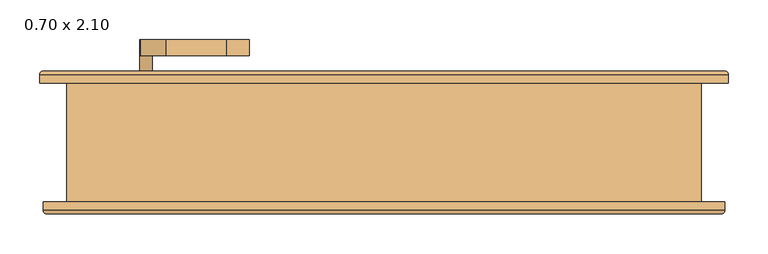
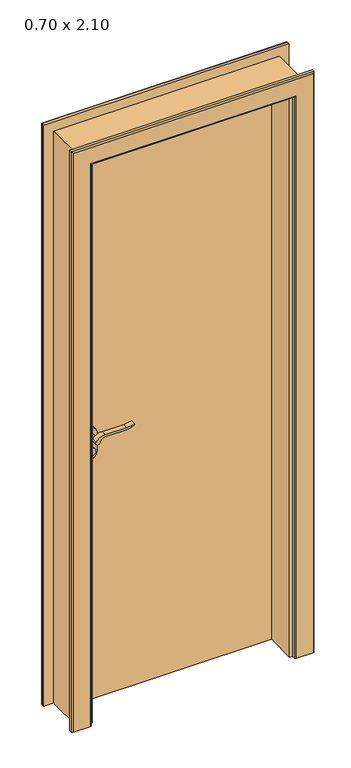
"""IFC4 building model written with IfcOpenShell, lengths in millimetres: door geometry, PORTA_DE_ABRIR_MADEIRA : 0.70 x 2.10."""

import ifcopenshell
import ifcopenshell.guid

model = None  # the IFC model being written
_history = None  # IfcOwnerHistory: only IFC2X3 demands one
_inside = {}  # id of a spatial element -> (the spatial element, [elements in it])
_under = {}  # id of a project, library or spatial element -> (it, [spatial elements below it])
_declared = {}  # id of a project -> (the project, [libraries it declares])
_typed = {}  # id of a type object -> (the type object, [elements of that type])
_made_of = {}  # id of a material, layer set ... -> (it, [elements and type objects made of it])


def new_model(schema):
    """Start an empty IFC model of exactly this schema.

    Asked for "IFC4X3", IfcOpenShell would pick the latest addendum, in which some entities
    have other attributes; the version numbers below select the first issue.
    IFC2X3 requires an IfcOwnerHistory on every rooted entity: one is made here for all.
    """
    global model, _history
    if schema == "IFC4X3":
        model = ifcopenshell.file(schema_version=(4, 3, 0, 0))
    else:
        model = ifcopenshell.file(schema=schema)
    _inside.clear()
    _under.clear()
    _declared.clear()
    _typed.clear()
    _made_of.clear()
    _history = None
    if model.schema == "IFC2X3":
        org = make("IfcOrganization", Name="unknown")
        user = make(
            "IfcPersonAndOrganization",
            ThePerson=make("IfcPerson", FamilyName="unknown"),
            TheOrganization=org,
        )
        app = make(
            "IfcApplication",
            ApplicationDeveloper=org,
            Version="unknown",
            ApplicationFullName="unknown",
            ApplicationIdentifier="unknown",
        )
        _history = make(
            "IfcOwnerHistory",
            OwningUser=user,
            OwningApplication=app,
            ChangeAction="ADDED",
            CreationDate=0,
        )
    return model


def make(cls, **values):
    """One entity of the class cls with the attributes given. An attribute that is None is left unset."""
    return model.create_entity(
        cls, **{name: value for name, value in values.items() if value is not None}
    )


def rooted(cls, **values):
    """An entity with a GlobalId (a new one), such as an element, a storey or a relation."""
    return make(cls, GlobalId=ifcopenshell.guid.new(), OwnerHistory=_history, **values)


def si_unit(unit_type, name, prefix=None):
    """IfcSIUnit, for example si_unit("LENGTHUNIT", "METRE", prefix="MILLI")."""
    return make("IfcSIUnit", UnitType=unit_type, Prefix=prefix, Name=name)


def assignment(units):
    """IfcUnitAssignment: the units of a project."""
    return None if units is None else make("IfcUnitAssignment", Units=units)


def point(xyz):
    """IfcCartesianPoint."""
    return None if xyz is None else make("IfcCartesianPoint", Coordinates=xyz)


def direction(xyz):
    """IfcDirection."""
    return None if xyz is None else make("IfcDirection", DirectionRatios=xyz)


def frame(location, z_axis=None, x_axis=None):
    """IfcAxis2Placement3D, a coordinate frame: its origin and axes. An axis left out is left unset."""
    return make(
        "IfcAxis2Placement3D",
        Location=point(location),
        Axis=direction(z_axis),
        RefDirection=direction(x_axis),
    )


def frame_2d(location, x_axis=None):
    """IfcAxis2Placement2D, a coordinate frame in the plane: its origin and x axis."""
    return make(
        "IfcAxis2Placement2D", Location=point(location), RefDirection=direction(x_axis)
    )


def origin():
    """The frame at (0, 0, 0) with its axes left unset."""
    return frame((0.0, 0.0, 0.0))


def origin_with_axes():
    """The frame at (0, 0, 0) with the z axis (0, 0, 1) and the x axis (1, 0, 0) written out."""
    return frame((0.0, 0.0, 0.0), z_axis=(0.0, 0.0, 1.0), x_axis=(1.0, 0.0, 0.0))


def place(relative_to, where):
    """IfcLocalPlacement: puts the frame where relative to a parent placement (None: the world)."""
    return make(
        "IfcLocalPlacement", PlacementRelTo=relative_to, RelativePlacement=where
    )


def context(
    kind, dimensions, precision=None, world=None, true_north=None, identifier=None
):
    """IfcGeometricRepresentationContext, for example the 3D "Model" context."""
    return make(
        "IfcGeometricRepresentationContext",
        ContextIdentifier=identifier,
        ContextType=kind,
        CoordinateSpaceDimension=dimensions,
        Precision=precision,
        WorldCoordinateSystem=world,
        TrueNorth=true_north,
    )


def project(units=None, contexts=None):
    """IfcProject with its units and contexts."""
    return rooted(
        "IfcProject",
        Name="project",
        RepresentationContexts=contexts,
        UnitsInContext=assignment(units),
    )


def spatial(cls, under=None, at=None, **own):
    """A site, building, storey or space (cls), placed at a placement, below another one or the project."""
    s = rooted(cls, ObjectPlacement=at, **own)
    if under is not None:
        _under.setdefault(under.id(), (under, []))[1].append(s)
    return s


def polyline(points):
    """IfcPolyline through the points."""
    return make("IfcPolyline", Points=[point(p) for p in points])


def circle_curve(where, radius):
    """IfcCircle in the frame where."""
    return make("IfcCircle", Position=where, Radius=radius)


def ellipse_curve(where, semi_axis1, semi_axis2):
    """IfcEllipse in the frame where."""
    return make(
        "IfcEllipse", Position=where, SemiAxis1=semi_axis1, SemiAxis2=semi_axis2
    )


def trimmed(basis, trim1, trim2, sense, master):
    """IfcTrimmedCurve: the piece of a basis curve between two trims."""
    return make(
        "IfcTrimmedCurve",
        BasisCurve=basis,
        Trim1=trim1,
        Trim2=trim2,
        SenseAgreement=sense,
        MasterRepresentation=master,
    )


def segment(curve, same_sense, transition):
    """IfcCompositeCurveSegment."""
    return make(
        "IfcCompositeCurveSegment",
        Transition=transition,
        SameSense=same_sense,
        ParentCurve=curve,
    )


def composite_curve(segments, self_intersect=None):
    """IfcCompositeCurve: segments joined end to end."""
    return make("IfcCompositeCurve", Segments=segments, SelfIntersect=self_intersect)


def outline(outer, holes=None, kind="AREA"):
    """IfcArbitraryClosedProfileDef: a profile drawn as a closed curve; with holes, ...WithVoids."""
    if holes is None:
        return make("IfcArbitraryClosedProfileDef", ProfileType=kind, OuterCurve=outer)
    return make(
        "IfcArbitraryProfileDefWithVoids",
        ProfileType=kind,
        OuterCurve=outer,
        InnerCurves=holes,
    )


def extrude(swept, where, along, depth):
    """IfcExtrudedAreaSolid: the profile swept, set in the frame where, extruded along a direction by depth."""
    return make(
        "IfcExtrudedAreaSolid",
        SweptArea=swept,
        Position=where,
        ExtrudedDirection=direction(along),
        Depth=depth,
    )


def faces_of(points, faces, orient=None, outer=None):
    """IfcFace entities. A face is a list of loops; a loop is a list of indices into points, from 0.

    orient and outer hold one flag for each loop. By default every Orientation is true, the
    first loop of a face is its IfcFaceOuterBound and the others are IfcFaceBound.
    """
    made = []
    for i, loops in enumerate(faces):
        bounds = []
        for j, loop in enumerate(loops):
            is_outer = j == 0 if outer is None else outer[i][j]
            bounds.append(
                make(
                    "IfcFaceOuterBound" if is_outer else "IfcFaceBound",
                    Bound=make("IfcPolyLoop", Polygon=[points[k] for k in loop]),
                    Orientation=True if orient is None else orient[i][j],
                )
            )
        made.append(make("IfcFace", Bounds=bounds))
    return made


def faceted_brep(points, faces, orient=None, outer=None, voids=None):
    """IfcFacetedBrep: a solid bounded by flat faces; with voids (closed shells), ...WithVoids."""
    shared = [point(p) for p in points]
    hull = make("IfcClosedShell", CfsFaces=faces_of(shared, faces, orient, outer))
    if voids is None:
        return make("IfcFacetedBrep", Outer=hull)
    return make(
        "IfcFacetedBrepWithVoids",
        Outer=hull,
        Voids=[
            make(cls, CfsFaces=faces_of(shared, fs, o, b)) for cls, fs, o, b in voids
        ],
    )


def shape(context_of_items, identifier, shape_type, items):
    """IfcShapeRepresentation: the items that make up one representation, for example the "Body"."""
    return make(
        "IfcShapeRepresentation",
        ContextOfItems=context_of_items,
        RepresentationIdentifier=identifier,
        RepresentationType=shape_type,
        Items=items,
    )


def source(mapping_origin, context_of_items, identifier, shape_type, items):
    """IfcRepresentationMap: a shape defined once, which mapped items show again and again."""
    return make(
        "IfcRepresentationMap",
        MappingOrigin=mapping_origin,
        MappedRepresentation=shape(context_of_items, identifier, shape_type, items),
    )


def transform(
    local_origin,
    x_axis=None,
    y_axis=None,
    z_axis=None,
    scale=None,
    scale2=None,
    scale3=None,
    uniform=True,
):
    """IfcCartesianTransformationOperator3D, or its non-uniform kind. x_axis, y_axis, z_axis: its Axis1, 2, 3."""
    if uniform:
        return make(
            "IfcCartesianTransformationOperator3D",
            Axis1=direction(x_axis),
            Axis2=direction(y_axis),
            LocalOrigin=point(local_origin),
            Scale=scale,
            Axis3=direction(z_axis),
        )
    return make(
        "IfcCartesianTransformationOperator3DnonUniform",
        Axis1=direction(x_axis),
        Axis2=direction(y_axis),
        LocalOrigin=point(local_origin),
        Scale=scale,
        Axis3=direction(z_axis),
        Scale2=scale2,
        Scale3=scale3,
    )


def mapped(mapping_source, mapping_target):
    """IfcMappedItem: shows the shape of a source again, moved by a transform."""
    return make(
        "IfcMappedItem", MappingSource=mapping_source, MappingTarget=mapping_target
    )


def made_of(thing, what):
    """Note that an element or type object is made of a material, layer set ...; save() writes the relation."""
    if what is not None:
        _made_of.setdefault(what.id(), (what, []))[1].append(thing)
    return thing


def element(
    cls,
    number,
    at=None,
    inside=None,
    cuts=None,
    type_object=None,
    material=None,
    context=None,
    identifier="Body",
    shape_type=None,
    held_by="IfcProductDefinitionShape",
    body=None,
    shapes=None,
    **own,
):
    """One element of the class cls, such as IfcWall. Its Tag is "e" and its number.

    at: its placement. inside: the storey or other place that contains it. cuts: it is an
    opening in that element (IfcRelVoidsElement). A single representation is given by context,
    identifier, shape_type and body (its items); several are given by shapes. held_by: the class
    of the entity that holds the representations. save() writes the other relations.
    """
    e = rooted(cls, Tag="e%d" % number, ObjectPlacement=at, **own)
    if body is not None:
        shapes = [shape(context, identifier, shape_type, body)]
    if shapes is not None:
        e.Representation = make(held_by, Representations=shapes)
    if inside is not None:
        _inside.setdefault(inside.id(), (inside, []))[1].append(e)
    if cuts is not None:
        rooted(
            "IfcRelVoidsElement", RelatingBuildingElement=cuts, RelatedOpeningElement=e
        )
    if type_object is not None:
        _typed.setdefault(type_object.id(), (type_object, []))[1].append(e)
    return made_of(e, material)


def aggregate(whole, parts):
    """IfcRelAggregates: a whole, such as a stair, and the parts it consists of."""
    return rooted("IfcRelAggregates", RelatingObject=whole, RelatedObjects=parts)


def save(model, path):
    """Write the relations noted so far, then the file.

    IfcRelAggregates (storeys below a building ...), IfcRelContainedInSpatialStructure (elements
    in a storey), IfcRelDefinesByType, IfcRelAssociatesMaterial and IfcRelDeclares: one each for
    every whole, place, type object, material and project.
    """
    for whole, parts in _under.values():
        aggregate(whole, parts)
    for where, things in _inside.values():
        rooted(
            "IfcRelContainedInSpatialStructure",
            RelatedElements=things,
            RelatingStructure=where,
        )
    for kind, things in _typed.values():
        rooted("IfcRelDefinesByType", RelatedObjects=things, RelatingType=kind)
    for what, things in _made_of.values():
        rooted("IfcRelAssociatesMaterial", RelatedObjects=things, RelatingMaterial=what)
    for by, libraries in _declared.values():
        rooted("IfcRelDeclares", RelatingContext=by, RelatedDefinitions=libraries)
    model.write(path)


def plane_surface(at):
    """IfcPlane: the flat surface through the origin of the frame at, square to its z axis."""
    return make("IfcPlane", Position=at)


def cylinder_surface(at, radius):
    """IfcCylindricalSurface: all points at the distance radius from the z axis of the frame at."""
    return make("IfcCylindricalSurface", Position=at, Radius=radius)


def advanced_brep(points, edges, surfaces, faces):
    """IfcAdvancedBrep: a solid bounded by faces that lie on surfaces and meet in shared edges.

    An edge is (start, end): straight between two places in points (the first is 0);
    or (start, end, curve); or (start, end, curve, False) where it runs against its curve.
    A face is (place in surfaces, loops), or (place, loops, False) where it looks against
    its surface's normal. A loop lists edges by number (the first is 1), with a minus sign
    where the edge is run from its end to its start. The first loop is the outer one.
    """
    corners = [point(p) for p in points]
    vertices = [make("IfcVertexPoint", VertexGeometry=c) for c in corners]
    made = []
    for start, end, *more in edges:
        made.append(
            make(
                "IfcEdgeCurve",
                EdgeStart=vertices[start],
                EdgeEnd=vertices[end],
                EdgeGeometry=more[0] if more else make("IfcPolyline", Points=[corners[start], corners[end]]),
                SameSense=more[1] if len(more) > 1 else True,
            )
        )
    hull = []
    for where, loops, *sense in faces:
        bounds = []
        for j, loop in enumerate(loops):
            ring = [make("IfcOrientedEdge", EdgeElement=made[abs(k) - 1], Orientation=k > 0) for k in loop]
            bounds.append(
                make(
                    "IfcFaceOuterBound" if j == 0 else "IfcFaceBound",
                    Bound=make("IfcEdgeLoop", EdgeList=ring),
                    Orientation=True,
                )
            )
        hull.append(make("IfcAdvancedFace", Bounds=bounds, FaceSurface=surfaces[where], SameSense=sense[0] if sense else True))
    return make("IfcAdvancedBrep", Outer=make("IfcClosedShell", CfsFaces=hull))


def door_0_70_x_2_10_357bc0c5(model_context):
    return source(origin(), model_context, "Body", "SolidModel", [
        extrude(outline(composite_curve([segment(trimmed(circle_curve(frame_2d((940.0, -300.0)), 15.0), [point((940.0, -285.0))], [point((940.0, -315.0))], False, "CARTESIAN"), True, "CONTINUOUS"), segment(trimmed(circle_curve(frame_2d((940.0, -300.0)), 15.0), [point((940.0, -315.0))], [point((940.0, -285.0))], False, "CARTESIAN"), True, "CONTINUOUS")], self_intersect=False)), frame((0.0, 15.0, 0.0), z_axis=(0.0, 1.0, 0.0), x_axis=(0.0, 0.0, 1.0)), (0.0, 0.0, 1.0), 10.0),
        extrude(outline(composite_curve([segment(trimmed(circle_curve(frame_2d((940.0, -300.0)), 15.0), [point((940.0, -285.0))], [point((940.0, -315.0))], False, "CARTESIAN"), True, "CONTINUOUS"), segment(trimmed(circle_curve(frame_2d((940.0, -300.0)), 15.0), [point((940.0, -315.0))], [point((940.0, -285.0))], False, "CARTESIAN"), True, "CONTINUOUS")], self_intersect=False)), frame((0.0, 80.0, 0.0), z_axis=(0.0, 1.0, 0.0), x_axis=(0.0, 0.0, 1.0)), (0.0, 0.0, 1.0), 10.0),
        extrude(outline(composite_curve([segment(trimmed(circle_curve(frame_2d((1000.0, -300.0)), 8.0), [point((1004.6523287, -306.5081363))], [point((1000.0, -292.0))], False, "CARTESIAN"), True, "CONTINUOUS"), segment(trimmed(circle_curve(frame_2d((994.8738613, -274.6138099)), 18.1261387), [point((1000.0, -292.0))], [point((1013.0, -274.6138099))], True, "CARTESIAN"), True, "CONTINUOUS"), segment(polyline([(1013.0, -274.6138099), (1013.0, -198.3564091)]), True, "CONTINUOUS"), segment(trimmed(circle_curve(frame_2d((1072.2709207, -201.9396612)), 59.3791355), [point((1013.0, -198.3564091))], [point((1022.2135558, -170.0))], False, "CARTESIAN"), True, "CONTINUOUS"), segment(polyline([(1022.2135558, -170.0), (1025.0, -170.0)]), True, "CONTINUOUS"), segment(trimmed(circle_curve(frame_2d((1103.2850638, -198.4227909)), 83.2850902), [point((1025.0, -170.0))], [point((1020.0, -198.3564091))], True, "CARTESIAN"), True, "CONTINUOUS"), segment(polyline([(1020.0, -198.3564091), (1020.0, -274.6325667)]), True, "CONTINUOUS"), segment(trimmed(circle_curve(frame_2d((982.7555521, -276.3324871)), 37.2832219), [point((1020.0, -274.6325667))], [point((1004.6523287, -306.5081363))], False, "CARTESIAN"), True, "CONTINUOUS")], self_intersect=False)), frame((0.0, -25.0, 0.0), z_axis=(0.0, 1.0, 0.0), x_axis=(0.0, 0.0, 1.0)), (0.0, 0.0, 1.0), 20.0),
        extrude(outline(composite_curve([segment(trimmed(circle_curve(frame_2d((994.8738682, -274.6138122)), 18.1261318), [point((999.9999903, -292.0))], [point((1013.0, -274.6138122))], True, "CARTESIAN"), True, "CONTINUOUS"), segment(polyline([(1013.0, -274.6138122), (1013.0, -198.3564091)]), True, "CONTINUOUS"), segment(trimmed(circle_curve(frame_2d((1072.2709207, -201.9396612)), 59.3791355), [point((1013.0, -198.3564091))], [point((1022.2135558, -170.0))], False, "CARTESIAN"), True, "CONTINUOUS"), segment(polyline([(1022.2135558, -170.0), (1025.0, -170.0)]), True, "CONTINUOUS"), segment(trimmed(circle_curve(frame_2d((1103.2850638, -198.4227909)), 83.2850902), [point((1025.0, -170.0))], [point((1020.0, -198.3564091))], True, "CARTESIAN"), True, "CONTINUOUS"), segment(polyline([(1020.0, -198.3564091), (1020.0, -274.6325667)]), True, "CONTINUOUS"), segment(trimmed(circle_curve(frame_2d((982.7555521, -276.3324871)), 37.2832219), [point((1020.0, -274.6325667))], [point((1004.6523287, -306.5081363))], False, "CARTESIAN"), True, "CONTINUOUS"), segment(trimmed(circle_curve(frame_2d((1000.0, -300.0)), 8.0), [point((1004.6523287, -306.5081363))], [point((999.9999903, -292.0))], False, "CARTESIAN"), True, "CONTINUOUS")], self_intersect=False)), frame((0.0, 110.0, 0.0), z_axis=(0.0, 1.0, 0.0), x_axis=(0.0, 0.0, 1.0)), (0.0, 0.0, 1.0), 20.0),
        extrude(outline(composite_curve([segment(trimmed(circle_curve(frame_2d((1000.0, -300.0)), 8.0), [point((1000.0, -292.0))], [point((1000.0, -308.0))], False, "CARTESIAN"), True, "CONTINUOUS"), segment(trimmed(circle_curve(frame_2d((1000.0, -300.0)), 8.0), [point((1000.0, -308.0))], [point((1000.0, -292.0))], False, "CARTESIAN"), True, "CONTINUOUS")], self_intersect=False)), frame((0.0, -5.0, 0.0), z_axis=(0.0, 1.0, 0.0), x_axis=(0.0, 0.0, 1.0)), (0.0, 0.0, 1.0), 30.0),
        extrude(outline(composite_curve([segment(trimmed(circle_curve(frame_2d((1000.0, -300.0)), 8.0), [point((1000.0, -292.0))], [point((1000.0, -308.0))], False, "CARTESIAN"), True, "CONTINUOUS"), segment(trimmed(circle_curve(frame_2d((1000.0, -300.0)), 8.0), [point((1000.0, -308.0))], [point((1000.0, -292.0))], False, "CARTESIAN"), True, "CONTINUOUS")], self_intersect=False)), frame((0.0, 80.0, 0.0), z_axis=(0.0, 1.0, 0.0), x_axis=(0.0, 0.0, 1.0)), (0.0, 0.0, 1.0), 30.0),
        extrude(outline(composite_curve([segment(trimmed(circle_curve(frame_2d((930.0, -300.0)), 25.0), [point((930.0, -325.0))], [point((930.0, -275.0))], False, "CARTESIAN"), True, "CONTINUOUS"), segment(polyline([(930.0, -275.0), (1000.0, -275.0)]), True, "CONTINUOUS"), segment(trimmed(circle_curve(frame_2d((1000.0, -300.0)), 25.0), [point((1000.0, -275.0))], [point((1000.0, -325.0))], False, "CARTESIAN"), True, "CONTINUOUS"), segment(polyline([(1000.0, -325.0), (930.0, -325.0)]), True, "CONTINUOUS")], self_intersect=False)), frame((0.0, 25.0, 0.0), z_axis=(0.0, 1.0, 0.0), x_axis=(0.0, 0.0, 1.0)), (0.0, 0.0, 1.0), 10.0),
        extrude(outline(composite_curve([segment(trimmed(circle_curve(frame_2d((930.0, -300.0)), 25.0), [point((930.0, -325.0))], [point((930.0, -275.0))], False, "CARTESIAN"), True, "CONTINUOUS"), segment(polyline([(930.0, -275.0), (1000.0, -275.0)]), True, "CONTINUOUS"), segment(trimmed(circle_curve(frame_2d((1000.0, -300.0)), 25.0), [point((1000.0, -275.0))], [point((1000.0, -325.0))], False, "CARTESIAN"), True, "CONTINUOUS"), segment(polyline([(1000.0, -325.0), (930.0, -325.0)]), True, "CONTINUOUS")], self_intersect=False)), frame((0.0, 70.0, 0.0), z_axis=(0.0, 1.0, 0.0), x_axis=(0.0, 0.0, 1.0)), (0.0, 0.0, 1.0), 10.0),
        faceted_brep([(-360.0, 35.0, 0.0), (-350.0, 35.0, 0.0), (-350.0, -75.0, 0.0), (-400.0, -75.0, 0.0), (-400.0, 75.0, 0.0), (-360.0, 75.0, 0.0), (-360.0, 75.0, 2100.0), (-360.0, 35.0, 2100.0), (-400.0, 75.0, 2140.0), (400.0, 75.0, 2140.0), (400.0, 75.0, 0.0), (360.0, 75.0, 0.0), (360.0, 75.0, 2100.0), (-400.0, -75.0, 2140.0), (-350.0, -75.0, 2090.0), (350.0, -75.0, 2090.0), (350.0, -75.0, 0.0), (400.0, -75.0, 0.0), (400.0, -75.0, 2140.0), (-350.0, 35.0, 2090.0), (360.0, 35.0, 2100.0), (360.0, 35.0, 0.0), (350.0, 35.0, 0.0), (350.0, 35.0, 2090.0)], [[[0, 1, 2, 3, 4, 5]], [[5, 6, 7, 0]], [[4, 8, 9, 10, 11, 12, 6, 5]], [[3, 13, 8, 4]], [[2, 14, 15, 16, 17, 18, 13, 3]], [[1, 19, 14, 2]], [[0, 7, 20, 21, 22, 23, 19, 1]], [[23, 22, 16, 15]], [[21, 11, 10, 17, 16, 22]], [[12, 11, 21, 20]], [[18, 17, 10, 9]], [[13, 18, 9, 8]], [[19, 23, 15, 14]], [[6, 12, 20, 7]]]),
        advanced_brep(
        [(-430.0, -75.3, 0.0), (-360.0, -75.3, 0.0), (-360.0, -85.3, 0.0), (-365.0, -90.3, 0.0), (-425.0, -90.3, 0.0), (-430.0, -85.3, 0.0), (-430.0, -85.3, 2170.0), (-430.0, -75.3, 2170.0), (-425.0, -90.3, 2165.0), (-365.0, -90.3, 2105.0), (365.0, -90.3, 2105.0), (365.0, -90.3, 0.0), (425.0, -90.3, 0.0), (425.0, -90.3, 2165.0), (-360.0, -85.3, 2100.0), (-360.0, -75.3, 2100.0), (430.0, -75.3, 2170.0), (430.0, -75.3, 0.0), (360.0, -75.3, 0.0), (360.0, -75.3, 2100.0), (430.0, -85.3, 0.0), (360.0, -85.3, 0.0), (360.0, -85.3, 2100.0), (430.0, -85.3, 2170.0)],
        [
            (0, 1),
            (1, 2),
            (2, 3, circle_curve(frame((-365.0, -85.3, 0.0), z_axis=(0.0, 0.0, -1.0), x_axis=(-1.0, 0.0, 0.0)), 5.0)),
            (3, 4),
            (4, 5, circle_curve(frame((-425.0, -85.3, 0.0), z_axis=(0.0, 0.0, -1.0), x_axis=(-1.0, 0.0, 0.0)), 5.0)),
            (5, 0),
            (5, 6),
            (6, 7),
            (7, 0),
            (4, 8),
            (8, 6, ellipse_curve(frame((-425.0, -85.3, 2165.0), z_axis=(-0.7071067811865475, 0.0, -0.7071067811865475), x_axis=(0.7071067811865474, 0.0, -0.7071067811865476)), 7.0710678, 5.0)),
            (3, 9),
            (9, 10),
            (10, 11),
            (11, 12),
            (12, 13),
            (13, 8),
            (2, 14),
            (14, 9, ellipse_curve(frame((-365.0, -85.3, 2105.0), z_axis=(-0.7071067811865475, 0.0, -0.7071067811865475), x_axis=(0.7071067811865474, 0.0, -0.7071067811865476)), 7.0710678, 5.0)),
            (1, 15),
            (15, 14),
            (7, 16),
            (16, 17),
            (17, 18),
            (18, 19),
            (19, 15),
            (17, 20),
            (20, 12, circle_curve(frame((425.0, -85.3, 0.0), z_axis=(0.0, 0.0, -1.0), x_axis=(1.0, 0.0, 0.0)), 5.0)),
            (11, 21, circle_curve(frame((365.0, -85.3, 0.0), z_axis=(0.0, 0.0, -1.0), x_axis=(1.0, 0.0, 0.0)), 5.0)),
            (21, 18),
            (21, 22),
            (22, 19),
            (10, 22, ellipse_curve(frame((365.0, -85.3, 2105.0), z_axis=(0.7071067811865475, 0.0, -0.7071067811865475), x_axis=(0.7071067811865474, 0.0, 0.7071067811865476)), 7.0710678, 5.0)),
            (20, 23),
            (23, 13, ellipse_curve(frame((425.0, -85.3, 2165.0), z_axis=(0.7071067811865475, 0.0, -0.7071067811865475), x_axis=(0.7071067811865474, 0.0, 0.7071067811865476)), 7.0710678, 5.0)),
            (16, 23),
            (6, 23),
            (22, 14),
        ],
        [
            plane_surface(frame((-400.0, 75.0, 0.0), z_axis=(0.0, 0.0, -1.0), x_axis=(0.0, 1.0, 0.0))),
            plane_surface(frame((-430.0, -75.3, 0.0), z_axis=(-1.0, 0.0, 0.0), x_axis=(0.0, 0.0, 1.0))),
            cylinder_surface(frame((-425.0, -85.3, 0.0), z_axis=(0.0, 0.0, -1.0), x_axis=(-1.0, 0.0, 0.0)), 5.0),
            plane_surface(frame((-425.0, -90.3, 0.0), z_axis=(0.0, -1.0, 0.0), x_axis=(0.0, 0.0, 1.0))),
            cylinder_surface(frame((-365.0, -85.3, 0.0), z_axis=(0.0, 0.0, -1.0), x_axis=(-1.0, 0.0, 0.0)), 5.0),
            plane_surface(frame((-360.0, -85.3, 0.0), z_axis=(1.0, 0.0, 0.0), x_axis=(0.0, 0.0, 1.0))),
            plane_surface(frame((-360.0, -75.3, 0.0), z_axis=(0.0, 1.0, 0.0), x_axis=(0.0, 0.0, 1.0))),
            plane_surface(frame((400.0, 75.0, 0.0), z_axis=(0.0, 0.0, -1.0), x_axis=(0.0, 1.0, 0.0))),
            plane_surface(frame((360.0, -85.3, 2100.0), z_axis=(-1.0, 0.0, 0.0), x_axis=(0.0, 0.0, -1.0))),
            cylinder_surface(frame((365.0, -85.3, 2140.0), z_axis=(0.0, 0.0, 1.0), x_axis=(1.0, 0.0, 0.0)), 5.0),
            cylinder_surface(frame((425.0, -85.3, 2140.0), z_axis=(0.0, 0.0, 1.0), x_axis=(1.0, 0.0, 0.0)), 5.0),
            plane_surface(frame((430.0, -75.3, 2170.0), z_axis=(1.0, 0.0, 0.0), x_axis=(0.0, 0.0, -1.0))),
            plane_surface(frame((-430.0, -75.3, 2170.0), z_axis=(0.0, 0.0, 1.0), x_axis=(1.0, 0.0, 0.0))),
            plane_surface(frame((-360.0, -85.3, 2100.0), z_axis=(0.0, 0.0, -1.0), x_axis=(1.0, 0.0, 0.0))),
            cylinder_surface(frame((-400.0, -85.3, 2165.0), z_axis=(-1.0, 0.0, 0.0), x_axis=(0.0, 0.0, 1.0)), 5.0),
            cylinder_surface(frame((-400.0, -85.3, 2105.0), z_axis=(-1.0, 0.0, 0.0), x_axis=(0.0, 0.0, 1.0)), 5.0),
        ],
        [
            (0, [[1, 2, 3, 4, 5, 6]]),
            (1, [[7, 8, 9, -6]]),
            (2, [[10, 11, -7, -5]]),
            (3, [[12, 13, 14, 15, 16, 17, -10, -4]]),
            (4, [[18, 19, -12, -3]]),
            (5, [[20, 21, -18, -2]]),
            (6, [[-9, 22, 23, 24, 25, 26, -20, -1]]),
            (7, [[27, 28, -15, 29, 30, -24]]),
            (8, [[-25, -30, 31, 32]]),
            (9, [[-31, -29, -14, 33]]),
            (10, [[-16, -28, 34, 35]]),
            (11, [[-34, -27, -23, 36]]),
            (12, [[37, -36, -22, -8]]),
            (13, [[-26, -32, 38, -21]]),
            (14, [[-17, -35, -37, -11]]),
            (15, [[-38, -33, -13, -19]]),
        ],
    ),
        advanced_brep(
        [(-429.3155593, 90.2647517, 0.0), (-369.3155593, 90.2647517, 0.0), (-364.3155593, 85.2647517, 0.0), (-364.3155593, 75.2647517, 0.0), (-434.3155593, 75.2647517, 0.0), (-434.3155593, 85.2647517, 0.0), (-434.3155593, 85.2647517, 2174.3155593), (-429.3155593, 90.2647517, 2169.3155593), (-434.3155593, 75.2647517, 2174.3155593), (-364.3155593, 75.2647517, 2104.3155593), (364.3155593, 75.2647517, 2104.3155593), (364.3155593, 75.2647517, 0.0), (434.3155593, 75.2647517, 0.0), (434.3155593, 75.2647517, 2174.3155593), (-364.3155593, 85.2647517, 2104.3155593), (-369.3155593, 90.2647517, 2109.3155593), (429.3155593, 90.2647517, 2169.3155593), (429.3155593, 90.2647517, 0.0), (369.3155593, 90.2647517, 0.0), (369.3155593, 90.2647517, 2109.3155593), (434.3155593, 85.2647517, 0.0), (364.3155593, 85.2647517, 0.0), (364.3155593, 85.2647517, 2104.3155593), (434.3155593, 85.2647517, 2174.3155593)],
        [
            (0, 1),
            (1, 2, circle_curve(frame((-369.3155593, 85.2647517, 0.0), z_axis=(0.0, 0.0, -1.0), x_axis=(-1.0, 0.0, 0.0)), 5.0)),
            (2, 3),
            (3, 4),
            (4, 5),
            (5, 0, circle_curve(frame((-429.3155593, 85.2647517, 0.0), z_axis=(0.0, 0.0, -1.0), x_axis=(-1.0, 0.0, 0.0)), 5.0)),
            (5, 6),
            (6, 7, ellipse_curve(frame((-429.3155593, 85.2647517, 2169.3155593), z_axis=(-0.7071067811865475, 0.0, -0.7071067811865475), x_axis=(0.7071067811865474, 0.0, -0.7071067811865476)), 7.0710678, 5.0)),
            (7, 0),
            (4, 8),
            (8, 6),
            (3, 9),
            (9, 10),
            (10, 11),
            (11, 12),
            (12, 13),
            (13, 8),
            (2, 14),
            (14, 9),
            (1, 15),
            (15, 14, ellipse_curve(frame((-369.3155593, 85.2647517, 2109.3155593), z_axis=(-0.7071067811865475, 0.0, -0.7071067811865475), x_axis=(0.7071067811865474, 0.0, -0.7071067811865476)), 7.0710678, 5.0)),
            (7, 16),
            (16, 17),
            (17, 18),
            (18, 19),
            (19, 15),
            (17, 20, circle_curve(frame((429.3155593, 85.2647517, 0.0), z_axis=(0.0, 0.0, -1.0), x_axis=(1.0, 0.0, 0.0)), 5.0)),
            (20, 12),
            (11, 21),
            (21, 18, circle_curve(frame((369.3155593, 85.2647517, 0.0), z_axis=(0.0, 0.0, -1.0), x_axis=(1.0, 0.0, 0.0)), 5.0)),
            (21, 22),
            (22, 19, ellipse_curve(frame((369.3155593, 85.2647517, 2109.3155593), z_axis=(0.7071067811865475, 0.0, -0.7071067811865475), x_axis=(0.7071067811865474, 0.0, 0.7071067811865476)), 7.0710678, 5.0)),
            (10, 22),
            (20, 23),
            (23, 13),
            (16, 23, ellipse_curve(frame((429.3155593, 85.2647517, 2169.3155593), z_axis=(0.7071067811865475, 0.0, -0.7071067811865475), x_axis=(0.7071067811865474, 0.0, 0.7071067811865476)), 7.0710678, 5.0)),
            (23, 6),
            (14, 22),
        ],
        [
            plane_surface(frame((-400.0, 75.0, 0.0), z_axis=(0.0, 0.0, -1.0), x_axis=(0.0, 1.0, 0.0))),
            cylinder_surface(frame((-429.3155593, 85.2647517, 0.0), z_axis=(0.0, 0.0, -1.0), x_axis=(-1.0, 0.0, 0.0)), 5.0),
            plane_surface(frame((-434.3155593, 85.2647517, 0.0), z_axis=(-1.0, 0.0, 0.0), x_axis=(0.0, 0.0, 1.0))),
            plane_surface(frame((-434.3155593, 75.2647517, 0.0), z_axis=(0.0, -1.0, 0.0), x_axis=(0.0, 0.0, 1.0))),
            plane_surface(frame((-364.3155593, 75.2647517, 0.0), z_axis=(1.0, 0.0, 0.0), x_axis=(0.0, 0.0, 1.0))),
            cylinder_surface(frame((-369.3155593, 85.2647517, 0.0), z_axis=(0.0, 0.0, -1.0), x_axis=(-1.0, 0.0, 0.0)), 5.0),
            plane_surface(frame((-369.3155593, 90.2647517, 0.0), z_axis=(0.0, 1.0, 0.0), x_axis=(0.0, 0.0, 1.0))),
            plane_surface(frame((400.0, 75.0, 0.0), z_axis=(0.0, 0.0, -1.0), x_axis=(0.0, 1.0, 0.0))),
            cylinder_surface(frame((369.3155593, 85.2647517, 2140.0), z_axis=(0.0, 0.0, 1.0), x_axis=(1.0, 0.0, 0.0)), 5.0),
            plane_surface(frame((364.3155593, 75.2647517, 2104.3155593), z_axis=(-1.0, 0.0, 0.0), x_axis=(0.0, 0.0, -1.0))),
            plane_surface(frame((434.3155593, 85.2647517, 2174.3155593), z_axis=(1.0, 0.0, 0.0), x_axis=(0.0, 0.0, -1.0))),
            cylinder_surface(frame((429.3155593, 85.2647517, 2140.0), z_axis=(0.0, 0.0, 1.0), x_axis=(1.0, 0.0, 0.0)), 5.0),
            plane_surface(frame((-434.3155593, 85.2647517, 2174.3155593), z_axis=(0.0, 0.0, 1.0), x_axis=(1.0, 0.0, 0.0))),
            plane_surface(frame((-364.3155593, 75.2647517, 2104.3155593), z_axis=(0.0, 0.0, -1.0), x_axis=(1.0, 0.0, 0.0))),
            cylinder_surface(frame((-400.0, 85.2647517, 2169.3155593), z_axis=(-1.0, 0.0, 0.0), x_axis=(0.0, 0.0, 1.0)), 5.0),
            cylinder_surface(frame((-400.0, 85.2647517, 2109.3155593), z_axis=(-1.0, 0.0, 0.0), x_axis=(0.0, 0.0, 1.0)), 5.0),
        ],
        [
            (0, [[1, 2, 3, 4, 5, 6]]),
            (1, [[7, 8, 9, -6]]),
            (2, [[10, 11, -7, -5]]),
            (3, [[12, 13, 14, 15, 16, 17, -10, -4]]),
            (4, [[18, 19, -12, -3]]),
            (5, [[20, 21, -18, -2]]),
            (6, [[-9, 22, 23, 24, 25, 26, -20, -1]]),
            (7, [[27, 28, -15, 29, 30, -24]]),
            (8, [[-25, -30, 31, 32]]),
            (9, [[-31, -29, -14, 33]]),
            (10, [[-16, -28, 34, 35]]),
            (11, [[-34, -27, -23, 36]]),
            (12, [[-17, -35, 37, -11]]),
            (13, [[38, -33, -13, -19]]),
            (14, [[-37, -36, -22, -8]]),
            (15, [[-26, -32, -38, -21]]),
        ],
    ),
        extrude(outline(polyline([(360.0, 70.0), (360.0, 35.0), (-360.0, 35.0), (-360.0, 70.0), (360.0, 70.0)])), origin_with_axes(), (0.0, 0.0, 1.0), 2100.0),
    ])


if __name__ == "__main__":
    model = new_model("IFC4")
    model_context = context("Model", 3, world=origin())
    ifc_project = project(units=[si_unit("LENGTHUNIT", "METRE", prefix="MILLI")], contexts=[model_context])
    site = spatial("IfcSite", under=ifc_project)
    building = spatial("IfcBuilding", under=site)
    placement = place(None, origin())
    door_0_70_x_2_10_shape = door_0_70_x_2_10_357bc0c5(model_context)
    element("IfcDoor", 1, ObjectType="PORTA_DE_ABRIR_MADEIRA : 0.70 x 2.10", at=placement, inside=building, context=model_context, shape_type="MappedRepresentation", body=[
        mapped(door_0_70_x_2_10_shape, transform((0.0, 0.0, 0.0), x_axis=(1.0, 0.0, 0.0), y_axis=(0.0, 1.0, 0.0), z_axis=(0.0, 0.0, 1.0))),
    ])
    save(model, "model.ifc")

# Revit data of these elements
# Type "PORTA_DE_ABRIR_MADEIRA : 0.70 x 2.10"
#   Type Mark = "P3"
#   Analytic Construction = "<Nenhum>"
#   Rough Width = 0.80 m
#   Projeção da estrutura externa = 0.025 m
#   Projeção da estrutura interna = 0.025 m
#   Largura da estrutura = 0.075 m
#   Rough Height = 2.15 m
#   Height = 2.10 m
#   Width = 0.70 m
#   Soleira [instance default] = no
#   Material do batente = .BATENTE E GUARNIÇÃO
#   Material da maçaneta = .AÇO INOXIDÁVEL ESCOVADO
#   Material da folha da porta = .FOLHA DA PORTA
#   Material da Soleira [instance default] = none
#   Function = (empty or 0)
#   Wall Closure = (empty or 0)
# Element 1 (IfcDoor, "PORTA_DE_ABRIR_MADEIRA : 0.70 x 2.10")
#   Materials on its faces: ".AÇO INOXIDÁVEL ESCOVADO", ".BATENTE E GUARNIÇÃO", ".FOLHA DA PORTA"
# Materials
#   ".BATENTE E GUARNIÇÃO": class "Madeira", colour RGB 215 186 156, transparency 0, Cost = 0
#   ".AÇO INOXIDÁVEL ESCOVADO": class "Metal", colour RGB 189 187 185, transparency 0, Description = "Stainless Steel 18/8, brushed finish", Cost = 0
#   ".FOLHA DA PORTA": class "Madeira", colour RGB 148 119 91, transparency 0, Cost = 0
